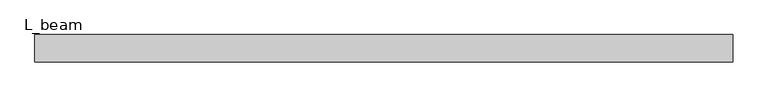
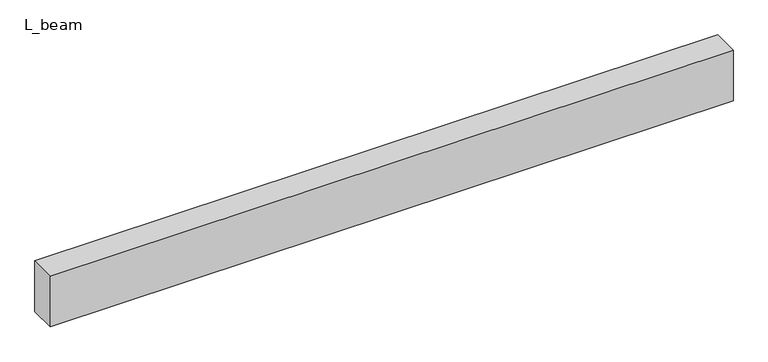
"""IFC4 building model written with IfcOpenShell, lengths in millimetres: beam geometry, 混凝土 - 矩形梁 : L_beam."""

import ifcopenshell
import ifcopenshell.guid

model = None  # the IFC model being written
_history = None  # IfcOwnerHistory: only IFC2X3 demands one
_inside = {}  # id of a spatial element -> (the spatial element, [elements in it])
_under = {}  # id of a project, library or spatial element -> (it, [spatial elements below it])
_declared = {}  # id of a project -> (the project, [libraries it declares])
_typed = {}  # id of a type object -> (the type object, [elements of that type])
_made_of = {}  # id of a material, layer set ... -> (it, [elements and type objects made of it])


def new_model(schema):
    """Start an empty IFC model of exactly this schema.

    Asked for "IFC4X3", IfcOpenShell would pick the latest addendum, in which some entities
    have other attributes; the version numbers below select the first issue.
    IFC2X3 requires an IfcOwnerHistory on every rooted entity: one is made here for all.
    """
    global model, _history
    if schema == "IFC4X3":
        model = ifcopenshell.file(schema_version=(4, 3, 0, 0))
    else:
        model = ifcopenshell.file(schema=schema)
    _inside.clear()
    _under.clear()
    _declared.clear()
    _typed.clear()
    _made_of.clear()
    _history = None
    if model.schema == "IFC2X3":
        org = make("IfcOrganization", Name="unknown")
        user = make(
            "IfcPersonAndOrganization",
            ThePerson=make("IfcPerson", FamilyName="unknown"),
            TheOrganization=org,
        )
        app = make(
            "IfcApplication",
            ApplicationDeveloper=org,
            Version="unknown",
            ApplicationFullName="unknown",
            ApplicationIdentifier="unknown",
        )
        _history = make(
            "IfcOwnerHistory",
            OwningUser=user,
            OwningApplication=app,
            ChangeAction="ADDED",
            CreationDate=0,
        )
    return model


def make(cls, **values):
    """One entity of the class cls with the attributes given. An attribute that is None is left unset."""
    return model.create_entity(
        cls, **{name: value for name, value in values.items() if value is not None}
    )


def rooted(cls, **values):
    """An entity with a GlobalId (a new one), such as an element, a storey or a relation."""
    return make(cls, GlobalId=ifcopenshell.guid.new(), OwnerHistory=_history, **values)


def si_unit(unit_type, name, prefix=None):
    """IfcSIUnit, for example si_unit("LENGTHUNIT", "METRE", prefix="MILLI")."""
    return make("IfcSIUnit", UnitType=unit_type, Prefix=prefix, Name=name)


def assignment(units):
    """IfcUnitAssignment: the units of a project."""
    return None if units is None else make("IfcUnitAssignment", Units=units)


def point(xyz):
    """IfcCartesianPoint."""
    return None if xyz is None else make("IfcCartesianPoint", Coordinates=xyz)


def direction(xyz):
    """IfcDirection."""
    return None if xyz is None else make("IfcDirection", DirectionRatios=xyz)


def frame(location, z_axis=None, x_axis=None):
    """IfcAxis2Placement3D, a coordinate frame: its origin and axes. An axis left out is left unset."""
    return make(
        "IfcAxis2Placement3D",
        Location=point(location),
        Axis=direction(z_axis),
        RefDirection=direction(x_axis),
    )


def origin():
    """The frame at (0, 0, 0) with its axes left unset."""
    return frame((0.0, 0.0, 0.0))


def place(relative_to, where):
    """IfcLocalPlacement: puts the frame where relative to a parent placement (None: the world)."""
    return make(
        "IfcLocalPlacement", PlacementRelTo=relative_to, RelativePlacement=where
    )


def context(
    kind, dimensions, precision=None, world=None, true_north=None, identifier=None
):
    """IfcGeometricRepresentationContext, for example the 3D "Model" context."""
    return make(
        "IfcGeometricRepresentationContext",
        ContextIdentifier=identifier,
        ContextType=kind,
        CoordinateSpaceDimension=dimensions,
        Precision=precision,
        WorldCoordinateSystem=world,
        TrueNorth=true_north,
    )


def project(units=None, contexts=None):
    """IfcProject with its units and contexts."""
    return rooted(
        "IfcProject",
        Name="project",
        RepresentationContexts=contexts,
        UnitsInContext=assignment(units),
    )


def spatial(cls, under=None, at=None, **own):
    """A site, building, storey or space (cls), placed at a placement, below another one or the project."""
    s = rooted(cls, ObjectPlacement=at, **own)
    if under is not None:
        _under.setdefault(under.id(), (under, []))[1].append(s)
    return s


def polyline(points):
    """IfcPolyline through the points."""
    return make("IfcPolyline", Points=[point(p) for p in points])


def outline(outer, holes=None, kind="AREA"):
    """IfcArbitraryClosedProfileDef: a profile drawn as a closed curve; with holes, ...WithVoids."""
    if holes is None:
        return make("IfcArbitraryClosedProfileDef", ProfileType=kind, OuterCurve=outer)
    return make(
        "IfcArbitraryProfileDefWithVoids",
        ProfileType=kind,
        OuterCurve=outer,
        InnerCurves=holes,
    )


def extrude(swept, where, along, depth):
    """IfcExtrudedAreaSolid: the profile swept, set in the frame where, extruded along a direction by depth."""
    return make(
        "IfcExtrudedAreaSolid",
        SweptArea=swept,
        Position=where,
        ExtrudedDirection=direction(along),
        Depth=depth,
    )


def shape(context_of_items, identifier, shape_type, items):
    """IfcShapeRepresentation: the items that make up one representation, for example the "Body"."""
    return make(
        "IfcShapeRepresentation",
        ContextOfItems=context_of_items,
        RepresentationIdentifier=identifier,
        RepresentationType=shape_type,
        Items=items,
    )


def source(mapping_origin, context_of_items, identifier, shape_type, items):
    """IfcRepresentationMap: a shape defined once, which mapped items show again and again."""
    return make(
        "IfcRepresentationMap",
        MappingOrigin=mapping_origin,
        MappedRepresentation=shape(context_of_items, identifier, shape_type, items),
    )


def transform(
    local_origin,
    x_axis=None,
    y_axis=None,
    z_axis=None,
    scale=None,
    scale2=None,
    scale3=None,
    uniform=True,
):
    """IfcCartesianTransformationOperator3D, or its non-uniform kind. x_axis, y_axis, z_axis: its Axis1, 2, 3."""
    if uniform:
        return make(
            "IfcCartesianTransformationOperator3D",
            Axis1=direction(x_axis),
            Axis2=direction(y_axis),
            LocalOrigin=point(local_origin),
            Scale=scale,
            Axis3=direction(z_axis),
        )
    return make(
        "IfcCartesianTransformationOperator3DnonUniform",
        Axis1=direction(x_axis),
        Axis2=direction(y_axis),
        LocalOrigin=point(local_origin),
        Scale=scale,
        Axis3=direction(z_axis),
        Scale2=scale2,
        Scale3=scale3,
    )


def mapped(mapping_source, mapping_target):
    """IfcMappedItem: shows the shape of a source again, moved by a transform."""
    return make(
        "IfcMappedItem", MappingSource=mapping_source, MappingTarget=mapping_target
    )


def made_of(thing, what):
    """Note that an element or type object is made of a material, layer set ...; save() writes the relation."""
    if what is not None:
        _made_of.setdefault(what.id(), (what, []))[1].append(thing)
    return thing


def element(
    cls,
    number,
    at=None,
    inside=None,
    cuts=None,
    type_object=None,
    material=None,
    context=None,
    identifier="Body",
    shape_type=None,
    held_by="IfcProductDefinitionShape",
    body=None,
    shapes=None,
    **own,
):
    """One element of the class cls, such as IfcWall. Its Tag is "e" and its number.

    at: its placement. inside: the storey or other place that contains it. cuts: it is an
    opening in that element (IfcRelVoidsElement). A single representation is given by context,
    identifier, shape_type and body (its items); several are given by shapes. held_by: the class
    of the entity that holds the representations. save() writes the other relations.
    """
    e = rooted(cls, Tag="e%d" % number, ObjectPlacement=at, **own)
    if body is not None:
        shapes = [shape(context, identifier, shape_type, body)]
    if shapes is not None:
        e.Representation = make(held_by, Representations=shapes)
    if inside is not None:
        _inside.setdefault(inside.id(), (inside, []))[1].append(e)
    if cuts is not None:
        rooted(
            "IfcRelVoidsElement", RelatingBuildingElement=cuts, RelatedOpeningElement=e
        )
    if type_object is not None:
        _typed.setdefault(type_object.id(), (type_object, []))[1].append(e)
    return made_of(e, material)


def aggregate(whole, parts):
    """IfcRelAggregates: a whole, such as a stair, and the parts it consists of."""
    return rooted("IfcRelAggregates", RelatingObject=whole, RelatedObjects=parts)


def save(model, path):
    """Write the relations noted so far, then the file.

    IfcRelAggregates (storeys below a building ...), IfcRelContainedInSpatialStructure (elements
    in a storey), IfcRelDefinesByType, IfcRelAssociatesMaterial and IfcRelDeclares: one each for
    every whole, place, type object, material and project.
    """
    for whole, parts in _under.values():
        aggregate(whole, parts)
    for where, things in _inside.values():
        rooted(
            "IfcRelContainedInSpatialStructure",
            RelatedElements=things,
            RelatingStructure=where,
        )
    for kind, things in _typed.values():
        rooted("IfcRelDefinesByType", RelatedObjects=things, RelatingType=kind)
    for what, things in _made_of.values():
        rooted("IfcRelAssociatesMaterial", RelatedObjects=things, RelatingMaterial=what)
    for by, libraries in _declared.values():
        rooted("IfcRelDeclares", RelatingContext=by, RelatedDefinitions=libraries)
    model.write(path)


def l_beam_c3390818(model_context):
    return source(origin(), model_context, "Body", "SweptSolid", [
        extrude(outline(polyline([(3826.0, 150.0), (3826.0, -150.0), (-3826.0, -150.0), (-3826.0, 150.0), (3826.0, 150.0)])), frame((0.0, 0.0, -300.0), z_axis=(0.0, 0.0, 1.0), x_axis=(1.0, 0.0, 0.0)), (0.0, 0.0, 1.0), 600.0),
    ])


if __name__ == "__main__":
    model = new_model("IFC4")
    model_context = context("Model", 3, world=origin())
    ifc_project = project(units=[si_unit("LENGTHUNIT", "METRE", prefix="MILLI")], contexts=[model_context])
    site = spatial("IfcSite", under=ifc_project)
    building = spatial("IfcBuilding", under=site)
    placement = place(None, origin())
    l_beam_shape = l_beam_c3390818(model_context)
    element("IfcBeam", 1, ObjectType="混凝土 - 矩形梁 : L_beam", at=placement, inside=building, context=model_context, shape_type="MappedRepresentation", body=[
        mapped(l_beam_shape, transform((0.0, 0.0, 0.0), x_axis=(1.0, 0.0, 0.0), y_axis=(0.0, 1.0, 0.0), z_axis=(0.0, 0.0, 1.0))),
    ])
    save(model, "model.ifc")

# Revit data of these elements
# Type "混凝土 - 矩形梁 : L_beam"
#   Length [instance default] = 1524 mm
#   b = 300 mm
#   h = 600 mm
#   Structural Material [instance default] = none
#   Assembly Code = ""
